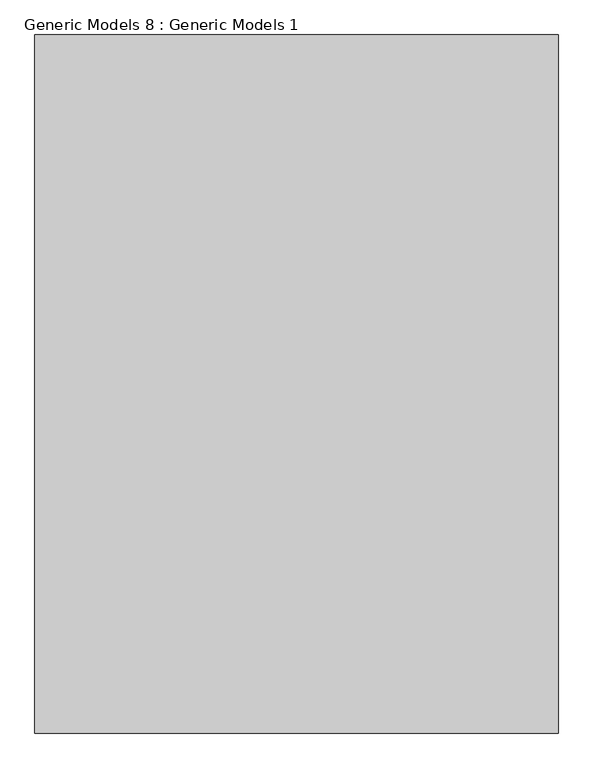
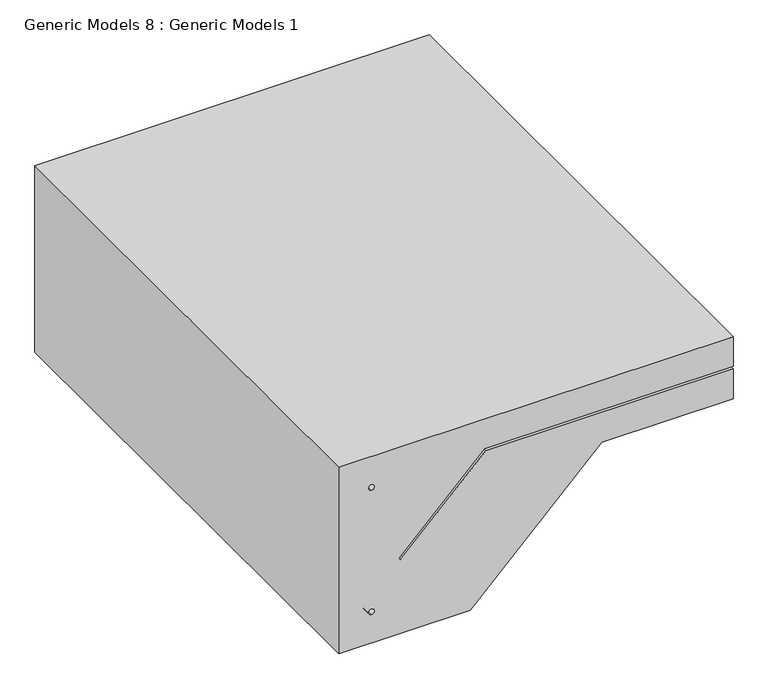
"""IFC4 building model written with IfcOpenShell, lengths in millimetres: proxy geometry, Generic Models 8 : Generic Models 1."""

from ifc_helpers import new_model, si_unit, point, frame, frame_2d, origin, place, context, project, spatial, polyline, circle_curve, trimmed, segment, composite_curve, outline, extrude, source, transform, mapped, element, save


def generic_models_8_generic_models_1_dd7fddfd(model_context):
    return source(origin(), model_context, "Body", "SweptSolid", [
        extrude(outline(polyline([(0.0, 52785.9625), (0.0, 51871.5625), (-457.2, 51871.5625), (-457.2, 52176.3625), (-152.4, 52481.1625), (-152.4, 52785.9625), (-79.375, 52785.9625), (-79.375, 52212.2583259), (-276.674432, 52014.9588939), (-272.1843039, 52010.4687659), (-73.025, 52209.6280698), (-73.025, 52785.9625), (0.0, 52785.9625)]), holes=[composite_curve([segment(trimmed(circle_curve(frame_2d((-76.2, 51947.7625)), 6.35), [point((-69.85, 51947.7625))], [point((-82.55, 51947.7625))], True, "CARTESIAN"), True, "CONTINUOUS"), segment(trimmed(circle_curve(frame_2d((-76.2, 51947.7625)), 6.35), [point((-82.55, 51947.7625))], [point((-69.85, 51947.7625))], True, "CARTESIAN"), True, "CONTINUOUS")], self_intersect=False), composite_curve([segment(trimmed(circle_curve(frame_2d((-381.0, 51947.7625)), 6.35), [point((-374.65, 51947.7625))], [point((-387.35, 51947.7625))], True, "CARTESIAN"), True, "CONTINUOUS"), segment(trimmed(circle_curve(frame_2d((-381.0, 51947.7625)), 6.35), [point((-387.35, 51947.7625))], [point((-374.65, 51947.7625))], True, "CARTESIAN"), True, "CONTINUOUS")], self_intersect=False)]), frame((0.0, 0.0, 0.0), z_axis=(0.0, 1.0, 0.0), x_axis=(0.0, 0.0, 1.0)), (0.0, 0.0, 1.0), 1219.2),
    ])


if __name__ == "__main__":
    model = new_model("IFC4")
    model_context = context("Model", 3, world=origin())
    ifc_project = project(units=[si_unit("LENGTHUNIT", "METRE", prefix="MILLI")], contexts=[model_context])
    site = spatial("IfcSite", under=ifc_project)
    building = spatial("IfcBuilding", under=site)
    placement = place(None, origin())
    generic_models_8_generic_models_1_shape = generic_models_8_generic_models_1_dd7fddfd(model_context)
    element("IfcBuildingElementProxy", 1, Name="Generic Models 8 : Generic Models 1", ObjectType="Generic Models 8 : Generic Models 1", at=placement, inside=building, context=model_context, shape_type="MappedRepresentation", body=[
        mapped(generic_models_8_generic_models_1_shape, transform((0.0, 0.0, 0.0), x_axis=(1.0, 0.0, 0.0), y_axis=(0.0, 1.0, 0.0), z_axis=(0.0, 0.0, 1.0))),
    ])
    save(model, "model.ifc")

# Revit data of these elements
# Element 1 (IfcBuildingElementProxy, "Generic Models 8 : Generic Models 1")
#   Materials on its faces: "CONCRETE (3000 PSI CONCRETE)", "#10 6x6 WIRE MESH", "#4 CONT. STEEL REBAR"
# Materials
#   "CONCRETE (3000 PSI CONCRETE)": class "Concrete", colour RGB 192 192 192, transparency 0, Description = "Cast-in-place concrete", Cost = 0
#   "#10 6x6 WIRE MESH": class "Metal", colour RGB 189 187 185, transparency 0, Description = "Structural steel 50ksi", Cost = 0
#   "#4 CONT. STEEL REBAR": class "Metal", colour RGB 189 187 185, transparency 0, Description = "Structural steel 50ksi", Cost = 0
